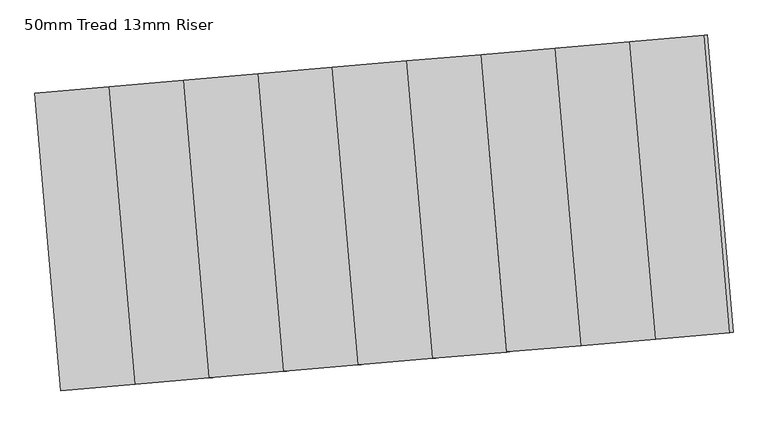
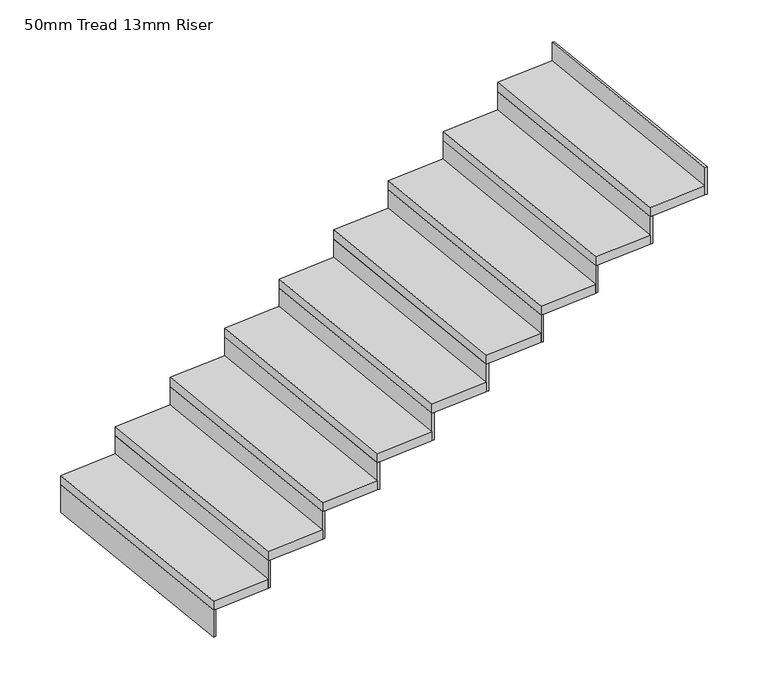
"""IFC4 building model written with IfcOpenShell, lengths in millimetres: stair flight geometry, 50mm Tread 13mm Riser."""

from ifc_helpers import new_model, si_unit, frame, origin, place, context, project, spatial, polyline, outline, extrude, source, transform, mapped, element, save


def stair_flight_50mm_tread_13mm_riser_7f78ee21(model_context):
    return source(origin(), model_context, "Body", "SweptSolid", [
        extrude(outline(polyline([(-14523.7337331, 13653.5141844), (-14536.187045, 13652.434822), (-14639.8058389, 14847.9527623), (-14627.352527, 14849.0321247), (-14523.7337331, 13653.5141844)])), frame((0.0, 0.0, 1450.0), z_axis=(0.0, 0.0, 1.0), x_axis=(1.0, 0.0, 0.0)), (0.0, 0.0, 1.0), 150.0),
        extrude(outline(polyline([(-14340.9263538, 14873.8574608), (-14237.3075599, 13678.3395205), (-14536.187045, 13652.434822), (-14639.8058389, 14847.9527623), (-14340.9263538, 14873.8574608)])), frame((0.0, 0.0, 1600.0), z_axis=(0.0, 0.0, 1.0), x_axis=(1.0, 0.0, 0.0)), (0.0, 0.0, 1.0), 50.0),
        extrude(outline(polyline([(-14224.854248, 13679.4188829), (-14237.3075599, 13678.3395205), (-14340.9263538, 14873.8574608), (-14328.473042, 14874.9368232), (-14224.854248, 13679.4188829)])), frame((0.0, 0.0, 1600.0), z_axis=(0.0, 0.0, 1.0), x_axis=(1.0, 0.0, 0.0)), (0.0, 0.0, 1.0), 150.0),
        extrude(outline(polyline([(-14042.0468688, 14899.7621593), (-13938.4280748, 13704.244219), (-14237.3075599, 13678.3395205), (-14340.9263538, 14873.8574608), (-14042.0468688, 14899.7621593)])), frame((0.0, 0.0, 1750.0), z_axis=(0.0, 0.0, 1.0), x_axis=(1.0, 0.0, 0.0)), (0.0, 0.0, 1.0), 50.0),
        extrude(outline(polyline([(-13925.9747629, 13705.3235814), (-13938.4280748, 13704.244219), (-14042.0468688, 14899.7621593), (-14029.5935569, 14900.8415217), (-13925.9747629, 13705.3235814)])), frame((0.0, 0.0, 1750.0), z_axis=(0.0, 0.0, 1.0), x_axis=(1.0, 0.0, 0.0)), (0.0, 0.0, 1.0), 150.0),
        extrude(outline(polyline([(-13743.1673837, 14925.6668578), (-13639.5485898, 13730.1489175), (-13938.4280748, 13704.244219), (-14042.0468688, 14899.7621593), (-13743.1673837, 14925.6668578)])), frame((0.0, 0.0, 1900.0), z_axis=(0.0, 0.0, 1.0), x_axis=(1.0, 0.0, 0.0)), (0.0, 0.0, 1.0), 50.0),
        extrude(outline(polyline([(-13627.0952779, 13731.2282799), (-13639.5485898, 13730.1489175), (-13743.1673837, 14925.6668578), (-13730.7140718, 14926.7462202), (-13627.0952779, 13731.2282799)])), frame((0.0, 0.0, 1900.0), z_axis=(0.0, 0.0, 1.0), x_axis=(1.0, 0.0, 0.0)), (0.0, 0.0, 1.0), 150.0),
        extrude(outline(polyline([(-13444.2878986, 14951.5715562), (-13340.6691047, 13756.053616), (-13639.5485898, 13730.1489175), (-13743.1673837, 14925.6668578), (-13444.2878986, 14951.5715562)])), frame((0.0, 0.0, 2050.0), z_axis=(0.0, 0.0, 1.0), x_axis=(1.0, 0.0, 0.0)), (0.0, 0.0, 1.0), 50.0),
        extrude(outline(polyline([(-13328.2157928, 13757.1329784), (-13340.6691047, 13756.053616), (-13444.2878986, 14951.5715562), (-13431.8345868, 14952.6509187), (-13328.2157928, 13757.1329784)])), frame((0.0, 0.0, 2050.0), z_axis=(0.0, 0.0, 1.0), x_axis=(1.0, 0.0, 0.0)), (0.0, 0.0, 1.0), 150.0),
        extrude(outline(polyline([(-13145.4084136, 14977.4762547), (-13041.7896196, 13781.9583144), (-13340.6691047, 13756.053616), (-13444.2878986, 14951.5715562), (-13145.4084136, 14977.4762547)])), frame((0.0, 0.0, 2200.0), z_axis=(0.0, 0.0, 1.0), x_axis=(1.0, 0.0, 0.0)), (0.0, 0.0, 1.0), 50.0),
        extrude(outline(polyline([(-13029.3363077, 13783.0376769), (-13041.7896196, 13781.9583144), (-13145.4084136, 14977.4762547), (-13132.9551017, 14978.5556172), (-13029.3363077, 13783.0376769)])), frame((0.0, 0.0, 2200.0), z_axis=(0.0, 0.0, 1.0), x_axis=(1.0, 0.0, 0.0)), (0.0, 0.0, 1.0), 150.0),
        extrude(outline(polyline([(-12846.5289285, 15003.3809532), (-12742.9101345, 13807.8630129), (-13041.7896196, 13781.9583144), (-13145.4084136, 14977.4762547), (-12846.5289285, 15003.3809532)])), frame((0.0, 0.0, 2350.0), z_axis=(0.0, 0.0, 1.0), x_axis=(1.0, 0.0, 0.0)), (0.0, 0.0, 1.0), 50.0),
        extrude(outline(polyline([(-12730.4568227, 13808.9423754), (-12742.9101345, 13807.8630129), (-12846.5289285, 15003.3809532), (-12834.0756166, 15004.4603157), (-12730.4568227, 13808.9423754)])), frame((0.0, 0.0, 2350.0), z_axis=(0.0, 0.0, 1.0), x_axis=(1.0, 0.0, 0.0)), (0.0, 0.0, 1.0), 150.0),
        extrude(outline(polyline([(-12547.6494434, 15029.2856517), (-12444.0306495, 13833.7677114), (-12742.9101345, 13807.8630129), (-12846.5289285, 15003.3809532), (-12547.6494434, 15029.2856517)])), frame((0.0, 0.0, 2500.0), z_axis=(0.0, 0.0, 1.0), x_axis=(1.0, 0.0, 0.0)), (0.0, 0.0, 1.0), 50.0),
        extrude(outline(polyline([(-12431.5773376, 13834.8470739), (-12444.0306495, 13833.7677114), (-12547.6494434, 15029.2856517), (-12535.1961315, 15030.3650141), (-12431.5773376, 13834.8470739)])), frame((0.0, 0.0, 2500.0), z_axis=(0.0, 0.0, 1.0), x_axis=(1.0, 0.0, 0.0)), (0.0, 0.0, 1.0), 150.0),
        extrude(outline(polyline([(-12248.7699583, 15055.1903502), (-12145.1511644, 13859.6724099), (-12444.0306495, 13833.7677114), (-12547.6494434, 15029.2856517), (-12248.7699583, 15055.1903502)])), frame((0.0, 0.0, 2650.0), z_axis=(0.0, 0.0, 1.0), x_axis=(1.0, 0.0, 0.0)), (0.0, 0.0, 1.0), 50.0),
        extrude(outline(polyline([(-12132.6978525, 13860.7517723), (-12145.1511644, 13859.6724099), (-12248.7699583, 15055.1903502), (-12236.3166465, 15056.2697126), (-12132.6978525, 13860.7517723)])), frame((0.0, 0.0, 2650.0), z_axis=(0.0, 0.0, 1.0), x_axis=(1.0, 0.0, 0.0)), (0.0, 0.0, 1.0), 150.0),
        extrude(outline(polyline([(-11833.8183674, 13886.6564708), (-11846.2716793, 13885.5771084), (-11949.8904733, 15081.0950487), (-11937.4371614, 15082.1744111), (-11833.8183674, 13886.6564708)])), frame((0.0, 0.0, 2800.0), z_axis=(0.0, 0.0, 1.0), x_axis=(1.0, 0.0, 0.0)), (0.0, 0.0, 1.0), 150.0),
        extrude(outline(polyline([(-11949.8904733, 15081.0950487), (-11846.2716793, 13885.5771084), (-12145.1511644, 13859.6724099), (-12248.7699583, 15055.1903502), (-11949.8904733, 15081.0950487)])), frame((0.0, 0.0, 2800.0), z_axis=(0.0, 0.0, 1.0), x_axis=(1.0, 0.0, 0.0)), (0.0, 0.0, 1.0), 50.0),
    ])


if __name__ == "__main__":
    model = new_model("IFC4")
    model_context = context("Model", 3, world=origin())
    ifc_project = project(units=[si_unit("LENGTHUNIT", "METRE", prefix="MILLI")], contexts=[model_context])
    site = spatial("IfcSite", under=ifc_project)
    building = spatial("IfcBuilding", under=site)
    placement = place(None, origin())
    stair_flight_50mm_tread_13mm_riser_shape = stair_flight_50mm_tread_13mm_riser_7f78ee21(model_context)
    element("IfcStairFlight", 1, ObjectType="50mm Tread 13mm Riser", at=placement, inside=building, context=model_context, shape_type="MappedRepresentation", body=[
        mapped(stair_flight_50mm_tread_13mm_riser_shape, transform((0.0, 0.0, 0.0), x_axis=(1.0, 0.0, 0.0), y_axis=(0.0, 1.0, 0.0), z_axis=(0.0, 0.0, 1.0))),
    ])
    save(model, "model.ifc")
